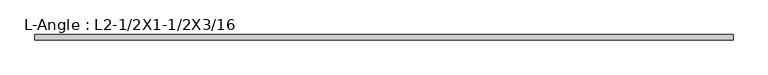
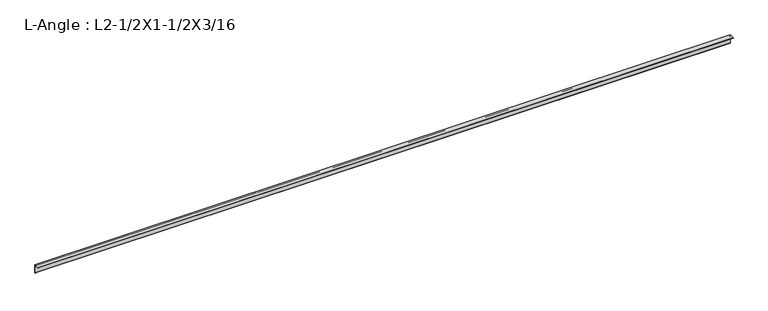
"""IFC4 building model written with IfcOpenShell, lengths in millimetres: beam geometry, L-Angle : L2-1/2X1-1/2X3/16."""

from ifc_helpers import new_model, si_unit, point, frame, frame_2d, origin, place, context, project, spatial, polyline, circle_curve, trimmed, segment, composite_curve, outline, extrude, source, transform, mapped, element, save


def l_angle_l2_1_2x1_1_2x3_16_55f30a5d(model_context):
    return source(origin(), model_context, "Body", "SweptSolid", [
        extrude(outline(composite_curve([segment(polyline([(8.8138, 21.3106), (8.8138, -42.1894)]), True, "CONTINUOUS"), segment(trimmed(circle_curve(frame_2d((8.8138, -37.4269)), 4.7625), [point((8.8138, -42.1894))], [point((4.0513, -37.4269))], False, "CARTESIAN"), True, "CONTINUOUS"), segment(polyline([(4.0513, -37.4269), (4.0513, 11.7856)]), True, "CONTINUOUS"), segment(trimmed(circle_curve(frame_2d((-0.7112, 11.7856)), 4.7625), [point((4.0513, 11.7856))], [point((-0.7112, 16.5481))], True, "CARTESIAN"), True, "CONTINUOUS"), segment(polyline([(-0.7112, 16.5481), (-24.5237, 16.5481)]), True, "CONTINUOUS"), segment(trimmed(circle_curve(frame_2d((-24.5237, 21.3106)), 4.7625), [point((-24.5237, 16.5481))], [point((-29.2862, 21.3106))], False, "CARTESIAN"), True, "CONTINUOUS"), segment(polyline([(-29.2862, 21.3106), (8.8138, 21.3106)]), True, "CONTINUOUS")], self_intersect=False)), frame((-2661.4335871, 0.0, 0.0), z_axis=(1.0, 0.0, 0.0), x_axis=(0.0, 1.0, 0.0)), (0.0, 0.0, 1.0), 5056.7144486),
    ])


if __name__ == "__main__":
    model = new_model("IFC4")
    model_context = context("Model", 3, world=origin())
    ifc_project = project(units=[si_unit("LENGTHUNIT", "METRE", prefix="MILLI")], contexts=[model_context])
    site = spatial("IfcSite", under=ifc_project)
    building = spatial("IfcBuilding", under=site)
    placement = place(None, origin())
    l_angle_l2_1_2x1_1_2x3_16_shape = l_angle_l2_1_2x1_1_2x3_16_55f30a5d(model_context)
    element("IfcBeam", 1, ObjectType="L-Angle : L2-1/2X1-1/2X3/16", at=placement, inside=building, context=model_context, shape_type="MappedRepresentation", body=[
        mapped(l_angle_l2_1_2x1_1_2x3_16_shape, transform((0.0, 0.0, 0.0), x_axis=(1.0, 0.0, 0.0), y_axis=(0.0, 1.0, 0.0), z_axis=(0.0, 0.0, 1.0))),
    ])
    save(model, "model.ifc")

# Revit data of these elements
# Type "L-Angle : L2-1/2X1-1/2X3/16"
#   Assembly Code = "B10"
#   k = 0' - 0 7/16"
#   W = 2.47
#   Start Extension Calculation [instance default] = 10' - 0"
#   Start Extension [instance default] = -0' - 0 1/2"
#   End Extension Calculation [instance default] = 10' - 0"
#   End Extension [instance default] = -0' - 0 1/2"
#   Length [instance default] = 5' - 0"
#   b = 0' - 1 1/2"
#   d = 0' - 2 1/2"
#   t = 0' - 0 3/16"
#   x = 0' - 0.347"
#   y = 0' - 0.839"
#   A = 0.00496528 SF
#   Structural Material [instance default] = Metal - Steel - ASTM A36
# Element 1 (IfcBeam, "L-Angle : L2-1/2X1-1/2X3/16")
#   Materials on its faces: "Metal - Steel - ASTM A36"
# Materials
#   "Metal - Steel - ASTM A36": class "Metal", colour RGB 199 199 199, transparency 0
